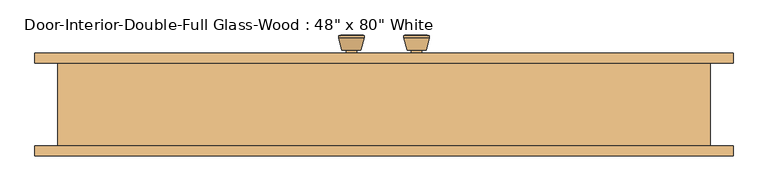
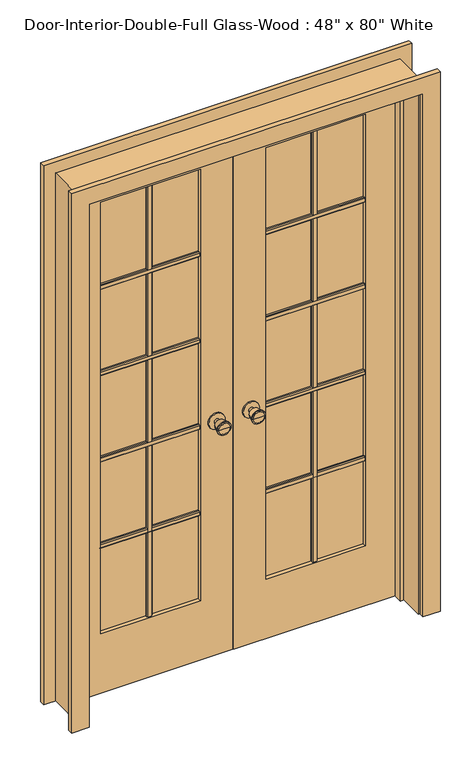
"""IFC4 building model written with IfcOpenShell, lengths in millimetres: door geometry."""

from ifc_helpers import new_model, si_unit, point, frame, frame_2d, origin, place, context, project, spatial, polyline, circle_curve, trimmed, segment, composite_curve, outline, extrude, faceted_brep, source, transform, mapped, element, save
from ifc_brep_helpers import plane_surface, cylinder_surface, revolved_surface, advanced_brep


def door_fc88373f(model_context):
    return source(origin(), model_context, "Body", "SolidModel", [
        advanced_brep(
        [(-63.5, 83.7875, 914.4), (-73.5, 83.7875, 914.4), (-53.5, 83.7875, 914.4), (-83.9758676, 132.7875, 914.4), (-63.5, 132.7875, 914.4), (-43.0241324, 132.7875, 914.4), (-88.5, 130.9596319, 914.4), (-38.5, 130.9596319, 914.4), (-88.5, 127.4959537, 914.4), (-38.5, 127.4959537, 914.4), (-82.136236, 102.7875, 914.4), (-44.863764, 102.7875, 914.4), (-73.5, 102.7875, 914.4), (-53.5, 102.7875, 914.4)],
        [
            (0, 1),
            (1, 2, circle_curve(frame((-63.5, 83.7875, 914.4), z_axis=(0.0, -1.0, 0.0), x_axis=(1.0, 0.0, 0.0)), 10.0)),
            (2, 0),
            (2, 1, circle_curve(frame((-63.5, 83.7875, 914.4), z_axis=(0.0, -1.0, 0.0), x_axis=(1.0, 0.0, 0.0)), 10.0)),
            (3, 4),
            (4, 5),
            (5, 3, circle_curve(frame((-63.5, 132.7875, 914.4), z_axis=(0.0, 1.0, 0.0), x_axis=(1.0, 0.0, 0.0)), 20.4758676)),
            (3, 5, circle_curve(frame((-63.5, 132.7875, 914.4), z_axis=(0.0, 1.0, 0.0), x_axis=(1.0, 0.0, 0.0)), 20.4758676)),
            (6, 3),
            (5, 7),
            (7, 6, circle_curve(frame((-63.5, 130.9596319, 914.4), z_axis=(0.0, 1.0, 0.0), x_axis=(1.0, 0.0, 0.0)), 25.0)),
            (6, 7, circle_curve(frame((-63.5, 130.9596319, 914.4), z_axis=(0.0, 1.0, 0.0), x_axis=(1.0, 0.0, 0.0)), 25.0)),
            (8, 6),
            (7, 9),
            (9, 8, circle_curve(frame((-63.5, 127.4959537, 914.4), z_axis=(0.0, 1.0, 0.0), x_axis=(1.0, 0.0, 0.0)), 25.0)),
            (8, 9, circle_curve(frame((-63.5, 127.4959537, 914.4), z_axis=(0.0, 1.0, 0.0), x_axis=(1.0, 0.0, 0.0)), 25.0)),
            (10, 8),
            (9, 11),
            (11, 10, circle_curve(frame((-63.5, 102.7875, 914.4), z_axis=(0.0, 1.0, 0.0), x_axis=(1.0, 0.0, 0.0)), 18.636236)),
            (10, 11, circle_curve(frame((-63.5, 102.7875, 914.4), z_axis=(0.0, 1.0, 0.0), x_axis=(1.0, 0.0, 0.0)), 18.636236)),
            (12, 10),
            (11, 13),
            (13, 12, circle_curve(frame((-63.5, 102.7875, 914.4), z_axis=(0.0, 1.0, 0.0), x_axis=(1.0, 0.0, 0.0)), 10.0)),
            (12, 13, circle_curve(frame((-63.5, 102.7875, 914.4), z_axis=(0.0, 1.0, 0.0), x_axis=(1.0, 0.0, 0.0)), 10.0)),
            (1, 12),
            (13, 2),
        ],
        [
            plane_surface(frame((-63.5, 83.7875, 914.4), z_axis=(0.0, -1.0, 0.0), x_axis=(1.0, 0.0, 0.0))),
            plane_surface(frame((-63.5, 132.7875, 914.4), z_axis=(0.0, 1.0, 0.0), x_axis=(1.0, 0.0, 0.0))),
            revolved_surface(polyline([(-43.0241324, 132.7875, 914.4), (-38.5, 130.9596319, 914.4)]), (-63.5, 83.7875, 914.4), (0.0, -1.0, 0.0)),
            cylinder_surface(frame((-63.5, 83.7875, 914.4), z_axis=(0.0, -1.0, 0.0), x_axis=(1.0, 0.0, 0.0)), 25.0),
            revolved_surface(polyline([(-38.5, 127.4959537, 914.4), (-44.863764, 102.7875, 914.4)]), (-63.5, 83.7875, 914.4), (0.0, -1.0, 0.0)),
            plane_surface(frame((-63.5, 102.7875, 914.4), z_axis=(0.0, -1.0, 0.0), x_axis=(1.0, 0.0, 0.0))),
            cylinder_surface(frame((-63.5, 83.7875, 914.4), z_axis=(0.0, -1.0, 0.0), x_axis=(1.0, 0.0, 0.0)), 10.0),
        ],
        [
            (0, [[1, 2, 3]]),
            (0, [[-3, 4, -1]]),
            (1, [[5, 6, 7]]),
            (1, [[-6, -5, 8]]),
            (2, [[9, -7, 10, 11]]),
            (2, [[-10, -8, -9, 12]]),
            (3, [[13, -11, 14, 15]]),
            (3, [[-14, -12, -13, 16]]),
            (4, [[17, -15, 18, 19]]),
            (4, [[-18, -16, -17, 20]]),
            (5, [[21, -19, 22, 23]]),
            (5, [[-22, -20, -21, 24]]),
            (6, [[25, -23, 26, -2]]),
            (6, [[-26, -24, -25, -4]]),
        ],
    ),
        extrude(outline(composite_curve([segment(trimmed(circle_curve(frame_2d((914.4, -63.5)), 30.0), [point((914.4, -33.5))], [point((914.4, -93.5))], False, "CARTESIAN"), True, "CONTINUOUS"), segment(trimmed(circle_curve(frame_2d((914.4, -63.5)), 30.0), [point((914.4, -93.5))], [point((914.4, -33.5))], False, "CARTESIAN"), True, "CONTINUOUS")], self_intersect=False)), frame((0.0, 77.7875, 0.0), z_axis=(0.0, 1.0, 0.0), x_axis=(0.0, 0.0, 1.0)), (0.0, 0.0, 1.0), 6.0),
        advanced_brep(
        [(-63.5, 36.8625, 914.4), (-53.5, 36.8625, 914.4), (-73.5, 36.8625, 914.4), (-83.9758676, -12.1375, 914.4), (-43.0241324, -12.1375, 914.4), (-63.5, -12.1375, 914.4), (-88.5, -10.3096319, 914.4), (-38.5, -10.3096319, 914.4), (-88.5, -6.8459537, 914.4), (-38.5, -6.8459537, 914.4), (-82.136236, 17.8625, 914.4), (-44.863764, 17.8625, 914.4), (-73.5, 17.8625, 914.4), (-53.5, 17.8625, 914.4)],
        [
            (0, 1),
            (1, 2, circle_curve(frame((-63.5, 36.8625, 914.4), z_axis=(0.0, 1.0, 0.0), x_axis=(1.0, 0.0, 0.0)), 10.0)),
            (2, 0),
            (2, 1, circle_curve(frame((-63.5, 36.8625, 914.4), z_axis=(0.0, 1.0, 0.0), x_axis=(1.0, 0.0, 0.0)), 10.0)),
            (3, 4, circle_curve(frame((-63.5, -12.1375, 914.4), z_axis=(0.0, -1.0, 0.0), x_axis=(1.0, 0.0, 0.0)), 20.4758676)),
            (4, 5),
            (5, 3),
            (4, 3, circle_curve(frame((-63.5, -12.1375, 914.4), z_axis=(0.0, -1.0, 0.0), x_axis=(1.0, 0.0, 0.0)), 20.4758676)),
            (6, 7, circle_curve(frame((-63.5, -10.3096319, 914.4), z_axis=(0.0, -1.0, 0.0), x_axis=(1.0, 0.0, 0.0)), 25.0)),
            (7, 4),
            (3, 6),
            (7, 6, circle_curve(frame((-63.5, -10.3096319, 914.4), z_axis=(0.0, -1.0, 0.0), x_axis=(1.0, 0.0, 0.0)), 25.0)),
            (8, 9, circle_curve(frame((-63.5, -6.8459537, 914.4), z_axis=(0.0, -1.0, 0.0), x_axis=(1.0, 0.0, 0.0)), 25.0)),
            (9, 7),
            (6, 8),
            (9, 8, circle_curve(frame((-63.5, -6.8459537, 914.4), z_axis=(0.0, -1.0, 0.0), x_axis=(1.0, 0.0, 0.0)), 25.0)),
            (10, 11, circle_curve(frame((-63.5, 17.8625, 914.4), z_axis=(0.0, -1.0, 0.0), x_axis=(1.0, 0.0, 0.0)), 18.636236)),
            (11, 9),
            (8, 10),
            (11, 10, circle_curve(frame((-63.5, 17.8625, 914.4), z_axis=(0.0, -1.0, 0.0), x_axis=(1.0, 0.0, 0.0)), 18.636236)),
            (12, 13, circle_curve(frame((-63.5, 17.8625, 914.4), z_axis=(0.0, -1.0, 0.0), x_axis=(1.0, 0.0, 0.0)), 10.0)),
            (13, 11),
            (10, 12),
            (13, 12, circle_curve(frame((-63.5, 17.8625, 914.4), z_axis=(0.0, -1.0, 0.0), x_axis=(1.0, 0.0, 0.0)), 10.0)),
            (1, 13),
            (12, 2),
        ],
        [
            plane_surface(frame((-63.5, 36.8625, 914.4), z_axis=(0.0, 1.0, 0.0), x_axis=(1.0, 0.0, 0.0))),
            plane_surface(frame((-63.5, -12.1375, 914.4), z_axis=(0.0, -1.0, 0.0), x_axis=(1.0, 0.0, 0.0))),
            revolved_surface(polyline([(-43.0241324, -12.1375, 914.4), (-38.5, -10.3096319, 914.4)]), (-63.5, 36.8625, 914.4), (0.0, 1.0, 0.0)),
            cylinder_surface(frame((-63.5, 36.8625, 914.4), z_axis=(0.0, 1.0, 0.0), x_axis=(1.0, 0.0, 0.0)), 25.0),
            revolved_surface(polyline([(-38.5, -6.8459537, 914.4), (-44.863764, 17.8625, 914.4)]), (-63.5, 36.8625, 914.4), (0.0, 1.0, 0.0)),
            plane_surface(frame((-63.5, 17.8625, 914.4), z_axis=(0.0, 1.0, 0.0), x_axis=(1.0, 0.0, 0.0))),
            cylinder_surface(frame((-63.5, 36.8625, 914.4), z_axis=(0.0, 1.0, 0.0), x_axis=(1.0, 0.0, 0.0)), 10.0),
        ],
        [
            (0, [[1, 2, 3]]),
            (0, [[-3, 4, -1]]),
            (1, [[5, 6, 7]]),
            (1, [[8, -7, -6]]),
            (2, [[9, 10, -5, 11]]),
            (2, [[12, -11, -8, -10]]),
            (3, [[13, 14, -9, 15]]),
            (3, [[16, -15, -12, -14]]),
            (4, [[17, 18, -13, 19]]),
            (4, [[20, -19, -16, -18]]),
            (5, [[21, 22, -17, 23]]),
            (5, [[24, -23, -20, -22]]),
            (6, [[-2, 25, -21, 26]]),
            (6, [[-4, -26, -24, -25]]),
        ],
    ),
        extrude(outline(composite_curve([segment(trimmed(circle_curve(frame_2d((914.4, -63.5)), 30.0), [point((914.4, -33.5))], [point((914.4, -93.5))], False, "CARTESIAN"), True, "CONTINUOUS"), segment(trimmed(circle_curve(frame_2d((914.4, -63.5)), 30.0), [point((914.4, -93.5))], [point((914.4, -33.5))], False, "CARTESIAN"), True, "CONTINUOUS")], self_intersect=False)), frame((0.0, 36.8625, 0.0), z_axis=(0.0, 1.0, 0.0), x_axis=(0.0, 0.0, 1.0)), (0.0, 0.0, 1.0), 6.0),
        extrude(outline(polyline([(56.8325, 1586.23), (56.8325, 1567.18), (50.4825, 1567.18), (47.3075, 1570.355), (47.3075, 1583.055), (50.4825, 1586.23), (56.8325, 1586.23)])), frame((120.65, 0.0, 0.0), z_axis=(1.0, 0.0, 0.0), x_axis=(0.0, 1.0, 0.0)), (0.0, 0.0, 1.0), 368.3),
        extrude(outline(polyline([(56.8325, 1249.9975), (56.8325, 1230.9475), (50.4825, 1230.9475), (47.3075, 1234.1225), (47.3075, 1246.8225), (50.4825, 1249.9975), (56.8325, 1249.9975)])), frame((120.65, 0.0, 0.0), z_axis=(1.0, 0.0, 0.0), x_axis=(0.0, 1.0, 0.0)), (0.0, 0.0, 1.0), 368.3),
        extrude(outline(polyline([(56.8325, 913.765), (56.8325, 894.715), (50.4825, 894.715), (47.3075, 897.89), (47.3075, 910.59), (50.4825, 913.765), (56.8325, 913.765)])), frame((120.65, 0.0, 0.0), z_axis=(1.0, 0.0, 0.0), x_axis=(0.0, 1.0, 0.0)), (0.0, 0.0, 1.0), 368.3),
        extrude(outline(polyline([(295.275, 56.8325), (314.325, 56.8325), (314.325, 50.4825), (311.15, 47.3075), (298.45, 47.3075), (295.275, 50.4825), (295.275, 56.8325)])), frame((0.0, 0.0, 231.775), z_axis=(0.0, 0.0, 1.0), x_axis=(1.0, 0.0, 0.0)), (0.0, 0.0, 1.0), 1681.1625),
        extrude(outline(polyline([(56.8325, 577.5325), (56.8325, 558.4825), (50.4825, 558.4825), (47.3075, 561.6575), (47.3075, 574.3575), (50.4825, 577.5325), (56.8325, 577.5325)])), frame((120.65, 0.0, 0.0), z_axis=(1.0, 0.0, 0.0), x_axis=(0.0, 1.0, 0.0)), (0.0, 0.0, 1.0), 368.3),
        extrude(outline(polyline([(63.8175, 1586.23), (70.1675, 1586.23), (73.3425, 1583.055), (73.3425, 1570.355), (70.1675, 1567.18), (63.8175, 1567.18), (63.8175, 1586.23)])), frame((-488.95, 0.0, 0.0), z_axis=(1.0, 0.0, 0.0), x_axis=(0.0, 1.0, 0.0)), (0.0, 0.0, 1.0), 368.3),
        extrude(outline(polyline([(63.8175, 1249.9975), (70.1675, 1249.9975), (73.3425, 1246.8225), (73.3425, 1234.1225), (70.1675, 1230.9475), (63.8175, 1230.9475), (63.8175, 1249.9975)])), frame((-488.95, 0.0, 0.0), z_axis=(1.0, 0.0, 0.0), x_axis=(0.0, 1.0, 0.0)), (0.0, 0.0, 1.0), 368.3),
        extrude(outline(polyline([(63.8175, 913.765), (70.1675, 913.765), (73.3425, 910.59), (73.3425, 897.89), (70.1675, 894.715), (63.8175, 894.715), (63.8175, 913.765)])), frame((-488.95, 0.0, 0.0), z_axis=(1.0, 0.0, 0.0), x_axis=(0.0, 1.0, 0.0)), (0.0, 0.0, 1.0), 368.3),
        extrude(outline(polyline([(-314.325, 63.8175), (-314.325, 70.1675), (-311.15, 73.3425), (-298.45, 73.3425), (-295.275, 70.1675), (-295.275, 63.8175), (-314.325, 63.8175)])), frame((0.0, 0.0, 231.775), z_axis=(0.0, 0.0, 1.0), x_axis=(1.0, 0.0, 0.0)), (0.0, 0.0, 1.0), 1681.1625),
        extrude(outline(polyline([(63.8175, 577.5325), (70.1675, 577.5325), (73.3425, 574.3575), (73.3425, 561.6575), (70.1675, 558.4825), (63.8175, 558.4825), (63.8175, 577.5325)])), frame((-488.95, 0.0, 0.0), z_axis=(1.0, 0.0, 0.0), x_axis=(0.0, 1.0, 0.0)), (0.0, 0.0, 1.0), 368.3),
        extrude(outline(polyline([(63.8175, 1586.23), (70.1675, 1586.23), (73.3425, 1583.055), (73.3425, 1570.355), (70.1675, 1567.18), (63.8175, 1567.18), (63.8175, 1586.23)])), frame((120.65, 0.0, 0.0), z_axis=(1.0, 0.0, 0.0), x_axis=(0.0, 1.0, 0.0)), (0.0, 0.0, 1.0), 368.3),
        extrude(outline(polyline([(63.8175, 1249.9975), (70.1675, 1249.9975), (73.3425, 1246.8225), (73.3425, 1234.1225), (70.1675, 1230.9475), (63.8175, 1230.9475), (63.8175, 1249.9975)])), frame((120.65, 0.0, 0.0), z_axis=(1.0, 0.0, 0.0), x_axis=(0.0, 1.0, 0.0)), (0.0, 0.0, 1.0), 368.3),
        extrude(outline(polyline([(63.8175, 913.765), (70.1675, 913.765), (73.3425, 910.59), (73.3425, 897.89), (70.1675, 894.715), (63.8175, 894.715), (63.8175, 913.765)])), frame((120.65, 0.0, 0.0), z_axis=(1.0, 0.0, 0.0), x_axis=(0.0, 1.0, 0.0)), (0.0, 0.0, 1.0), 368.3),
        extrude(outline(polyline([(295.275, 63.8175), (295.275, 70.1675), (298.45, 73.3425), (311.15, 73.3425), (314.325, 70.1675), (314.325, 63.8175), (295.275, 63.8175)])), frame((0.0, 0.0, 231.775), z_axis=(0.0, 0.0, 1.0), x_axis=(1.0, 0.0, 0.0)), (0.0, 0.0, 1.0), 1681.1625),
        extrude(outline(polyline([(63.8175, 577.5325), (70.1675, 577.5325), (73.3425, 574.3575), (73.3425, 561.6575), (70.1675, 558.4825), (63.8175, 558.4825), (63.8175, 577.5325)])), frame((120.65, 0.0, 0.0), z_axis=(1.0, 0.0, 0.0), x_axis=(0.0, 1.0, 0.0)), (0.0, 0.0, 1.0), 368.3),
        extrude(outline(polyline([(56.8325, 1586.23), (56.8325, 1567.18), (50.4825, 1567.18), (47.3075, 1570.355), (47.3075, 1583.055), (50.4825, 1586.23), (56.8325, 1586.23)])), frame((-488.95, 0.0, 0.0), z_axis=(1.0, 0.0, 0.0), x_axis=(0.0, 1.0, 0.0)), (0.0, 0.0, 1.0), 368.3),
        extrude(outline(polyline([(56.8325, 1249.9975), (56.8325, 1230.9475), (50.4825, 1230.9475), (47.3075, 1234.1225), (47.3075, 1246.8225), (50.4825, 1249.9975), (56.8325, 1249.9975)])), frame((-488.95, 0.0, 0.0), z_axis=(1.0, 0.0, 0.0), x_axis=(0.0, 1.0, 0.0)), (0.0, 0.0, 1.0), 368.3),
        extrude(outline(polyline([(56.8325, 913.765), (56.8325, 894.715), (50.4825, 894.715), (47.3075, 897.89), (47.3075, 910.59), (50.4825, 913.765), (56.8325, 913.765)])), frame((-488.95, 0.0, 0.0), z_axis=(1.0, 0.0, 0.0), x_axis=(0.0, 1.0, 0.0)), (0.0, 0.0, 1.0), 368.3),
        extrude(outline(polyline([(-314.325, 56.8325), (-295.275, 56.8325), (-295.275, 50.4825), (-298.45, 47.3075), (-311.15, 47.3075), (-314.325, 50.4825), (-314.325, 56.8325)])), frame((0.0, 0.0, 231.775), z_axis=(0.0, 0.0, 1.0), x_axis=(1.0, 0.0, 0.0)), (0.0, 0.0, 1.0), 1681.1625),
        extrude(outline(polyline([(56.8325, 577.5325), (56.8325, 558.4825), (50.4825, 558.4825), (47.3075, 561.6575), (47.3075, 574.3575), (50.4825, 577.5325), (56.8325, 577.5325)])), frame((-488.95, 0.0, 0.0), z_axis=(1.0, 0.0, 0.0), x_axis=(0.0, 1.0, 0.0)), (0.0, 0.0, 1.0), 368.3),
        advanced_brep(
        [(63.5, 36.8625, 914.4), (73.5, 36.8625, 914.4), (53.5, 36.8625, 914.4), (83.9758676, -12.1375, 914.4), (63.5, -12.1375, 914.4), (43.0241324, -12.1375, 914.4), (88.5, -10.3096319, 914.4), (38.5, -10.3096319, 914.4), (88.5, -6.8459537, 914.4), (38.5, -6.8459537, 914.4), (82.136236, 17.8625, 914.4), (44.863764, 17.8625, 914.4), (73.5, 17.8625, 914.4), (53.5, 17.8625, 914.4)],
        [
            (0, 1),
            (1, 2, circle_curve(frame((63.5, 36.8625, 914.4), z_axis=(0.0, 1.0, 0.0), x_axis=(-1.0, 0.0, 0.0)), 10.0)),
            (2, 0),
            (2, 1, circle_curve(frame((63.5, 36.8625, 914.4), z_axis=(0.0, 1.0, 0.0), x_axis=(-1.0, 0.0, 0.0)), 10.0)),
            (3, 4),
            (4, 5),
            (5, 3, circle_curve(frame((63.5, -12.1375, 914.4), z_axis=(0.0, -1.0, 0.0), x_axis=(-1.0, 0.0, 0.0)), 20.4758676)),
            (3, 5, circle_curve(frame((63.5, -12.1375, 914.4), z_axis=(0.0, -1.0, 0.0), x_axis=(-1.0, 0.0, 0.0)), 20.4758676)),
            (6, 3),
            (5, 7),
            (7, 6, circle_curve(frame((63.5, -10.3096319, 914.4), z_axis=(0.0, -1.0, 0.0), x_axis=(-1.0, 0.0, 0.0)), 25.0)),
            (6, 7, circle_curve(frame((63.5, -10.3096319, 914.4), z_axis=(0.0, -1.0, 0.0), x_axis=(-1.0, 0.0, 0.0)), 25.0)),
            (8, 6),
            (7, 9),
            (9, 8, circle_curve(frame((63.5, -6.8459537, 914.4), z_axis=(0.0, -1.0, 0.0), x_axis=(-1.0, 0.0, 0.0)), 25.0)),
            (8, 9, circle_curve(frame((63.5, -6.8459537, 914.4), z_axis=(0.0, -1.0, 0.0), x_axis=(-1.0, 0.0, 0.0)), 25.0)),
            (10, 8),
            (9, 11),
            (11, 10, circle_curve(frame((63.5, 17.8625, 914.4), z_axis=(0.0, -1.0, 0.0), x_axis=(-1.0, 0.0, 0.0)), 18.636236)),
            (10, 11, circle_curve(frame((63.5, 17.8625, 914.4), z_axis=(0.0, -1.0, 0.0), x_axis=(-1.0, 0.0, 0.0)), 18.636236)),
            (12, 10),
            (11, 13),
            (13, 12, circle_curve(frame((63.5, 17.8625, 914.4), z_axis=(0.0, -1.0, 0.0), x_axis=(-1.0, 0.0, 0.0)), 10.0)),
            (12, 13, circle_curve(frame((63.5, 17.8625, 914.4), z_axis=(0.0, -1.0, 0.0), x_axis=(-1.0, 0.0, 0.0)), 10.0)),
            (1, 12),
            (13, 2),
        ],
        [
            plane_surface(frame((63.5, 36.8625, 914.4), z_axis=(0.0, 1.0, 0.0), x_axis=(-1.0, 0.0, 0.0))),
            plane_surface(frame((63.5, -12.1375, 914.4), z_axis=(0.0, -1.0, 0.0), x_axis=(-1.0, 0.0, 0.0))),
            revolved_surface(polyline([(43.0241324, -12.1375, 914.4), (38.5, -10.3096319, 914.4)]), (63.5, 36.8625, 914.4), (0.0, 1.0, 0.0)),
            cylinder_surface(frame((63.5, 36.8625, 914.4), z_axis=(0.0, 1.0, 0.0), x_axis=(-1.0, 0.0, 0.0)), 25.0),
            revolved_surface(polyline([(38.5, -6.8459537, 914.4), (44.863764, 17.8625, 914.4)]), (63.5, 36.8625, 914.4), (0.0, 1.0, 0.0)),
            plane_surface(frame((63.5, 17.8625, 914.4), z_axis=(0.0, 1.0, 0.0), x_axis=(-1.0, 0.0, 0.0))),
            cylinder_surface(frame((63.5, 36.8625, 914.4), z_axis=(0.0, 1.0, 0.0), x_axis=(-1.0, 0.0, 0.0)), 10.0),
        ],
        [
            (0, [[1, 2, 3]]),
            (0, [[-3, 4, -1]]),
            (1, [[5, 6, 7]]),
            (1, [[-6, -5, 8]]),
            (2, [[9, -7, 10, 11]]),
            (2, [[-10, -8, -9, 12]]),
            (3, [[13, -11, 14, 15]]),
            (3, [[-14, -12, -13, 16]]),
            (4, [[17, -15, 18, 19]]),
            (4, [[-18, -16, -17, 20]]),
            (5, [[21, -19, 22, 23]]),
            (5, [[-22, -20, -21, 24]]),
            (6, [[25, -23, 26, -2]]),
            (6, [[-26, -24, -25, -4]]),
        ],
    ),
        extrude(outline(composite_curve([segment(trimmed(circle_curve(frame_2d((914.4, 63.5)), 30.0), [point((914.4, 33.5))], [point((914.4, 93.5))], False, "CARTESIAN"), True, "CONTINUOUS"), segment(trimmed(circle_curve(frame_2d((914.4, 63.5)), 30.0), [point((914.4, 93.5))], [point((914.4, 33.5))], False, "CARTESIAN"), True, "CONTINUOUS")], self_intersect=False)), frame((0.0, 36.8625, 0.0), z_axis=(0.0, 1.0, 0.0), x_axis=(0.0, 0.0, 1.0)), (0.0, 0.0, 1.0), 6.0),
        advanced_brep(
        [(63.5, 83.7875, 914.4), (53.5, 83.7875, 914.4), (73.5, 83.7875, 914.4), (83.9758676, 132.7875, 914.4), (43.0241324, 132.7875, 914.4), (63.5, 132.7875, 914.4), (88.5, 130.9596319, 914.4), (38.5, 130.9596319, 914.4), (88.5, 127.4959537, 914.4), (38.5, 127.4959537, 914.4), (82.136236, 102.7875, 914.4), (44.863764, 102.7875, 914.4), (73.5, 102.7875, 914.4), (53.5, 102.7875, 914.4)],
        [
            (0, 1),
            (1, 2, circle_curve(frame((63.5, 83.7875, 914.4), z_axis=(0.0, -1.0, 0.0), x_axis=(-1.0, 0.0, 0.0)), 10.0)),
            (2, 0),
            (2, 1, circle_curve(frame((63.5, 83.7875, 914.4), z_axis=(0.0, -1.0, 0.0), x_axis=(-1.0, 0.0, 0.0)), 10.0)),
            (3, 4, circle_curve(frame((63.5, 132.7875, 914.4), z_axis=(0.0, 1.0, 0.0), x_axis=(-1.0, 0.0, 0.0)), 20.4758676)),
            (4, 5),
            (5, 3),
            (4, 3, circle_curve(frame((63.5, 132.7875, 914.4), z_axis=(0.0, 1.0, 0.0), x_axis=(-1.0, 0.0, 0.0)), 20.4758676)),
            (6, 7, circle_curve(frame((63.5, 130.9596319, 914.4), z_axis=(0.0, 1.0, 0.0), x_axis=(-1.0, 0.0, 0.0)), 25.0)),
            (7, 4),
            (3, 6),
            (7, 6, circle_curve(frame((63.5, 130.9596319, 914.4), z_axis=(0.0, 1.0, 0.0), x_axis=(-1.0, 0.0, 0.0)), 25.0)),
            (8, 9, circle_curve(frame((63.5, 127.4959537, 914.4), z_axis=(0.0, 1.0, 0.0), x_axis=(-1.0, 0.0, 0.0)), 25.0)),
            (9, 7),
            (6, 8),
            (9, 8, circle_curve(frame((63.5, 127.4959537, 914.4), z_axis=(0.0, 1.0, 0.0), x_axis=(-1.0, 0.0, 0.0)), 25.0)),
            (10, 11, circle_curve(frame((63.5, 102.7875, 914.4), z_axis=(0.0, 1.0, 0.0), x_axis=(-1.0, 0.0, 0.0)), 18.636236)),
            (11, 9),
            (8, 10),
            (11, 10, circle_curve(frame((63.5, 102.7875, 914.4), z_axis=(0.0, 1.0, 0.0), x_axis=(-1.0, 0.0, 0.0)), 18.636236)),
            (12, 13, circle_curve(frame((63.5, 102.7875, 914.4), z_axis=(0.0, 1.0, 0.0), x_axis=(-1.0, 0.0, 0.0)), 10.0)),
            (13, 11),
            (10, 12),
            (13, 12, circle_curve(frame((63.5, 102.7875, 914.4), z_axis=(0.0, 1.0, 0.0), x_axis=(-1.0, 0.0, 0.0)), 10.0)),
            (1, 13),
            (12, 2),
        ],
        [
            plane_surface(frame((63.5, 83.7875, 914.4), z_axis=(0.0, -1.0, 0.0), x_axis=(-1.0, 0.0, 0.0))),
            plane_surface(frame((63.5, 132.7875, 914.4), z_axis=(0.0, 1.0, 0.0), x_axis=(-1.0, 0.0, 0.0))),
            revolved_surface(polyline([(43.0241324, 132.7875, 914.4), (38.5, 130.9596319, 914.4)]), (63.5, 83.7875, 914.4), (0.0, -1.0, 0.0)),
            cylinder_surface(frame((63.5, 83.7875, 914.4), z_axis=(0.0, -1.0, 0.0), x_axis=(-1.0, 0.0, 0.0)), 25.0),
            revolved_surface(polyline([(38.5, 127.4959537, 914.4), (44.863764, 102.7875, 914.4)]), (63.5, 83.7875, 914.4), (0.0, -1.0, 0.0)),
            plane_surface(frame((63.5, 102.7875, 914.4), z_axis=(0.0, -1.0, 0.0), x_axis=(-1.0, 0.0, 0.0))),
            cylinder_surface(frame((63.5, 83.7875, 914.4), z_axis=(0.0, -1.0, 0.0), x_axis=(-1.0, 0.0, 0.0)), 10.0),
        ],
        [
            (0, [[1, 2, 3]]),
            (0, [[-3, 4, -1]]),
            (1, [[5, 6, 7]]),
            (1, [[8, -7, -6]]),
            (2, [[9, 10, -5, 11]]),
            (2, [[12, -11, -8, -10]]),
            (3, [[13, 14, -9, 15]]),
            (3, [[16, -15, -12, -14]]),
            (4, [[17, 18, -13, 19]]),
            (4, [[20, -19, -16, -18]]),
            (5, [[21, 22, -17, 23]]),
            (5, [[24, -23, -20, -22]]),
            (6, [[-2, 25, -21, 26]]),
            (6, [[-4, -26, -24, -25]]),
        ],
    ),
        extrude(outline(composite_curve([segment(trimmed(circle_curve(frame_2d((914.4, 63.5)), 30.0), [point((914.4, 33.5))], [point((914.4, 93.5))], False, "CARTESIAN"), True, "CONTINUOUS"), segment(trimmed(circle_curve(frame_2d((914.4, 63.5)), 30.0), [point((914.4, 93.5))], [point((914.4, 33.5))], False, "CARTESIAN"), True, "CONTINUOUS")], self_intersect=False)), frame((0.0, 77.7875, 0.0), z_axis=(0.0, 1.0, 0.0), x_axis=(0.0, 0.0, 1.0)), (0.0, 0.0, 1.0), 6.0),
        extrude(outline(polyline([(0.0, 615.95), (0.0, 679.45), (2101.85, 679.45), (2101.85, -679.45), (0.0, -679.45), (0.0, -615.95), (2038.35, -615.95), (2038.35, 615.95), (0.0, 615.95)])), frame((0.0, 77.7875, 0.0), z_axis=(0.0, 1.0, 0.0), x_axis=(0.0, 0.0, 1.0)), (0.0, 0.0, 1.0), 19.05),
        extrude(outline(polyline([(0.0, 615.95), (0.0, 679.45), (2101.85, 679.45), (2101.85, -679.45), (0.0, -679.45), (0.0, -615.95), (2038.35, -615.95), (2038.35, 615.95), (0.0, 615.95)])), frame((0.0, -103.1875, 0.0), z_axis=(0.0, 1.0, 0.0), x_axis=(0.0, 0.0, 1.0)), (0.0, 0.0, 1.0), 19.05),
        extrude(outline(polyline([(2032.0, -609.6), (0.0, -609.6), (0.0, -1.6019111), (2032.0, -1.6019111), (2032.0, -609.6)]), holes=[polyline([(231.775, -488.95), (1912.9375, -488.95), (1912.9375, -120.65), (231.775, -120.65), (231.775, -488.95)])]), frame((0.0, 42.8625, 0.0), z_axis=(0.0, 1.0, 0.0), x_axis=(0.0, 0.0, 1.0)), (0.0, 0.0, 1.0), 34.925),
        extrude(outline(polyline([(0.0, 609.6), (2032.0, 609.6), (2032.0, 1.5875), (0.0, 1.5875), (0.0, 609.6)]), holes=[polyline([(1912.9375, 120.65), (1912.9375, 488.95), (231.775, 488.95), (231.775, 120.65), (1912.9375, 120.65)])]), frame((0.0, 42.8625, 0.0), z_axis=(0.0, 1.0, 0.0), x_axis=(0.0, 0.0, 1.0)), (0.0, 0.0, 1.0), 34.925),
        faceted_brep([(635.0, 77.7875, 0.0), (635.0, -84.1375, 0.0), (609.6, -84.1375, 0.0), (609.6, 7.9375, 0.0), (596.9, 7.9375, 0.0), (596.9, 42.8625, 0.0), (609.6, 42.8625, 0.0), (609.6, 77.7875, 0.0), (635.0, 77.7875, 2057.4), (635.0, -84.1375, 2057.4), (-635.0, -84.1375, 2057.4), (-635.0, -84.1375, 0.0), (-609.6, -84.1375, 0.0), (-609.6, -84.1375, 2032.0), (609.6, -84.1375, 2032.0), (609.6, 7.9375, 2032.0), (-609.6, 7.9375, 2032.0), (-609.6, 7.9375, 0.0), (-596.9, 7.9375, 0.0), (-596.9, 7.9375, 2019.3), (596.9, 7.9375, 2019.3), (596.9, 42.8625, 2019.3), (1.5875, 42.8625, 2019.3), (-1.6019111, 42.8625, 2019.3), (-596.9, 42.8625, 2019.3), (-596.9, 42.8625, 0.0), (-609.6, 42.8625, 0.0), (-609.6, 42.8625, 2032.0), (-1.6019111, 42.8625, 2032.0), (1.5875, 42.8625, 2032.0), (609.6, 42.8625, 2032.0), (609.6, 77.7875, 2032.0), (1.5875, 77.7875, 2032.0), (-1.6019111, 77.7875, 2032.0), (-609.6, 77.7875, 2032.0), (-609.6, 77.7875, 0.0), (-635.0, 77.7875, 0.0), (-635.0, 77.7875, 2057.4)], [[[0, 1, 2, 3, 4, 5, 6, 7]], [[1, 0, 8, 9]], [[2, 1, 9, 10, 11, 12, 13, 14]], [[3, 2, 14, 15]], [[4, 3, 15, 16, 17, 18, 19, 20]], [[5, 4, 20, 21]], [[6, 5, 21, 22, 23, 24, 25, 26, 27, 28, 29, 30]], [[7, 6, 30, 31]], [[0, 7, 31, 32, 33, 34, 35, 36, 37, 8]], [[9, 8, 37, 10]], [[14, 13, 16, 15]], [[20, 19, 24, 23, 22, 21]], [[31, 30, 29, 28, 27, 34, 33, 32]], [[12, 11, 36, 35, 26, 25, 18, 17]], [[11, 10, 37, 36]], [[13, 12, 17, 16]], [[19, 18, 25, 24]], [[27, 26, 35, 34]]]),
        extrude(outline(polyline([(488.95, 56.8325), (120.65, 56.8325), (120.65, 63.8175), (488.95, 63.8175), (488.95, 56.8325)])), frame((0.0, 0.0, 231.775), z_axis=(0.0, 0.0, 1.0), x_axis=(1.0, 0.0, 0.0)), (0.0, 0.0, 1.0), 1681.1625),
        extrude(outline(polyline([(-120.65, 56.8325), (-488.95, 56.8325), (-488.95, 63.8175), (-120.65, 63.8175), (-120.65, 56.8325)])), frame((0.0, 0.0, 231.775), z_axis=(0.0, 0.0, 1.0), x_axis=(1.0, 0.0, 0.0)), (0.0, 0.0, 1.0), 1681.1625),
    ])


if __name__ == "__main__":
    model = new_model("IFC4")
    model_context = context("Model", 3, world=origin())
    ifc_project = project(units=[si_unit("LENGTHUNIT", "METRE", prefix="MILLI")], contexts=[model_context])
    site = spatial("IfcSite", under=ifc_project)
    building = spatial("IfcBuilding", under=site)
    placement = place(None, origin())
    door_shape = door_fc88373f(model_context)
    element("IfcDoor", 1, ObjectType="Door-Interior-Double-Full Glass-Wood : 48\" x 80\" White", at=placement, inside=building, context=model_context, shape_type="MappedRepresentation", body=[
        mapped(door_shape, transform((0.0, 0.0, 0.0), x_axis=(1.0, 0.0, 0.0), y_axis=(0.0, 1.0, 0.0), z_axis=(0.0, 0.0, 1.0))),
    ])
    save(model, "model.ifc")

# Revit data of these elements
# Type "Door-Interior-Double-Full Glass-Wood : 48\" x 80\" White"
#   Type Mark = "63"
#   COBie.Type.CreatedBy = "doug.wood@us.ibm.com"
#   COBie.Type.CreatedOn = "2016-04-14T02:07:24"
#   COBie.Type.Name = "Doors_Door-Interior-Double-Full Glass-Wood_48\" x 80\" White_63"
#   COBie.Type.Category = "23-30 10 00 : Doors"
#   COBie.Type.Description = "Door-Interior-Double-Full Glass-Wood_48\" x 80\" White"
#   COBie.Type.Manufacturer = ""
#   COBie.Type.ModelNumber = ""
#   Assembly Code = "C1020300"
#   Analytic Construction = "French door, wood frame with single glass"
#   COBie.Type.ReplacementCost = 0
#   Top Rail = 0' - 4 11/16"
#   Thickness = 0' - 1 3/8"
#   Thermal Resistance (R) = 0.188367 (m²·K)/W
#   Swing Angle [instance default] = 90.00°
#   Stiles = 0' - 4 3/4"
#   Rough Width = 4' - 2"
#   Rough Height = 6' - 9"
#   Panel Width = 2' - 0"
#   Height = 6' - 8"
#   Width = 4' - 0"
#   Heat Transfer Coefficient (U) = 5.30918 W/(m²·K)
#   Bottom Rail = 0' - 9 1/8"
#   COBie.Type = no
#   Show Grill [instance default] = yes
#   Trim Material = Trim - White
#   Panel Material = Door - Panel
#   Frame Material = Door - Panel
#   Door Handle Material = Aluminum
#   Visual Light Transmittance = 0
#   Solar Heat Gain Coefficient = 0
#   Wall Closure = (empty or 0)
#   Function = (empty or 0)
# Element 1 (IfcDoor, "Door-Interior-Double-Full Glass-Wood : 48\" x 80\" White")
#   Materials on its faces: "Door - Panel", "Aluminum", "Trim - White", "Glass"
# Materials
#   "Trim - White": class "Wood", colour RGB 255 255 255, transparency 0, Cost = 0
#   "Door - Panel": class "Wood", colour RGB 255 255 255, transparency 0, Cost = 0
#   "Aluminum": class "Metal", colour RGB 247 247 247, transparency 0, Description = "Aluminum 6061", Cost = 0
#   "Glass": class "Glass", colour RGB 0 128 192, transparency 0.75, Description = "Soda Lime Glass", Cost = 0
